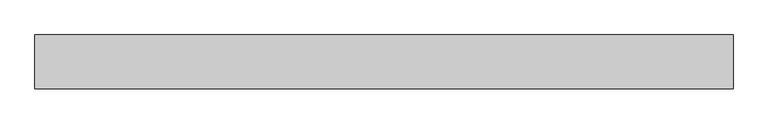
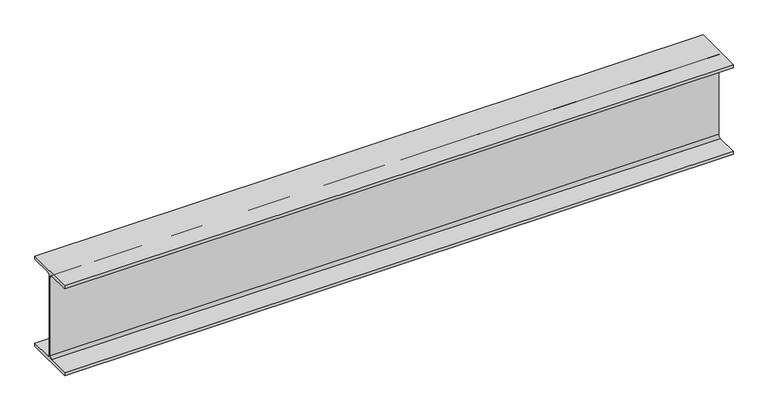
"""IFC4 building model written with IfcOpenShell, lengths in millimetres: beam geometry, Steel Beam_H-KSD3502 : H_SB_ASB_H-194x150x6x9."""

from ifc_helpers import new_model, si_unit, point, frame, frame_2d, origin, place, context, project, spatial, polyline, circle_curve, trimmed, segment, composite_curve, outline, extrude, source, transform, mapped, element, save


def beam_825be00d(model_context):
    return source(origin(), model_context, "Body", "SweptSolid", [
        extrude(outline(composite_curve([segment(polyline([(-82.5, -141.5), (-11.9, -141.5)]), True, "CONTINUOUS"), segment(trimmed(circle_curve(frame_2d((-11.9, -132.6)), 8.9), [point((-11.9, -141.5))], [point((-3.0, -132.6))], True, "CARTESIAN"), True, "CONTINUOUS"), segment(polyline([(-3.0, -132.6), (-3.0, 132.6)]), True, "CONTINUOUS"), segment(trimmed(circle_curve(frame_2d((-11.9, 132.6)), 8.9), [point((-3.0, 132.6))], [point((-11.9, 141.5))], True, "CARTESIAN"), True, "CONTINUOUS"), segment(polyline([(-11.9, 141.5), (-82.5, 141.5), (-82.5, 151.7), (82.5, 151.7), (82.5, 141.5), (11.9, 141.5)]), True, "CONTINUOUS"), segment(trimmed(circle_curve(frame_2d((11.9, 132.6)), 8.9), [point((11.9, 141.5))], [point((3.0, 132.6))], True, "CARTESIAN"), True, "CONTINUOUS"), segment(polyline([(3.0, 132.6), (3.0, -132.6)]), True, "CONTINUOUS"), segment(trimmed(circle_curve(frame_2d((11.9, -132.6)), 8.9), [point((3.0, -132.6))], [point((11.9, -141.5))], True, "CARTESIAN"), True, "CONTINUOUS"), segment(polyline([(11.9, -141.5), (82.5, -141.5), (82.5, -151.7), (-82.5, -151.7), (-82.5, -141.5)]), True, "CONTINUOUS")], self_intersect=False)), frame((-1067.7446443, 0.0, 0.0), z_axis=(1.0, 0.0, 0.0), x_axis=(0.0, 1.0, 0.0)), (0.0, 0.0, 1.0), 2135.4892885),
    ])


if __name__ == "__main__":
    model = new_model("IFC4")
    model_context = context("Model", 3, world=origin())
    ifc_project = project(units=[si_unit("LENGTHUNIT", "METRE", prefix="MILLI")], contexts=[model_context])
    site = spatial("IfcSite", under=ifc_project)
    building = spatial("IfcBuilding", under=site)
    placement = place(None, origin())
    beam_shape = beam_825be00d(model_context)
    element("IfcBeam", 1, ObjectType="Steel Beam_H-KSD3502 : H_SB_ASB_H-194x150x6x9", at=placement, inside=building, context=model_context, shape_type="MappedRepresentation", body=[
        mapped(beam_shape, transform((0.0, 0.0, 0.0), x_axis=(1.0, 0.0, 0.0), y_axis=(0.0, 1.0, 0.0), z_axis=(0.0, 0.0, 1.0))),
    ])
    save(model, "model.ifc")

# Revit data of these elements
# Type "Steel Beam_H-KSD3502 : H_SB_ASB_H-194x150x6x9"
#   Width = 15.0 cm
#   Web Thickness = 0.6 cm
#   Web Fillet = 1.3 cm
#   Warping Constant = 43316.0 cm⁶
#   Torsional Moment of Inertia = 8.622 cm⁴
#   Torsional Modulus = 1.0 cm³
#   Section Area = 39.01 cm²
#   Plastic Modulus weak axis = 104.0 cm³
#   Plastic Modulus strong axis = 309.0 cm³
#   Perimeter = 0.95 m²/m
#   Nominal Weight = 30.60 kgf/m
#   Moment of Inertia weak axis = 507.00 cm⁴
#   Moment of Inertia strong axis = 2690.00 cm⁴
#   Height = 19.4 cm
#   Flange Thickness = 0.9 cm
#   Elastic Modulus weak axis = 67.6 cm³
#   Elastic Modulus strong axis = 277.0 cm³
#   Centroid Vertical = 9.7 cm
#   Centroid Horizontal = 7.5 cm
#   Length [instance default] = 1.5240 m
#   Structural Material [instance default] = Steel, 45-345
#   Assembly Code = ""
# Element 1 (IfcBeam, "Steel Beam_H-KSD3502 : H_SB_ASB_H-194x150x6x9")
#   Structural Material = none
# Materials
#   "Steel, 45-345": class "Metal", colour RGB 189 187 185, transparency 0, Description = "Steel 345 MPa", Cost = 0
